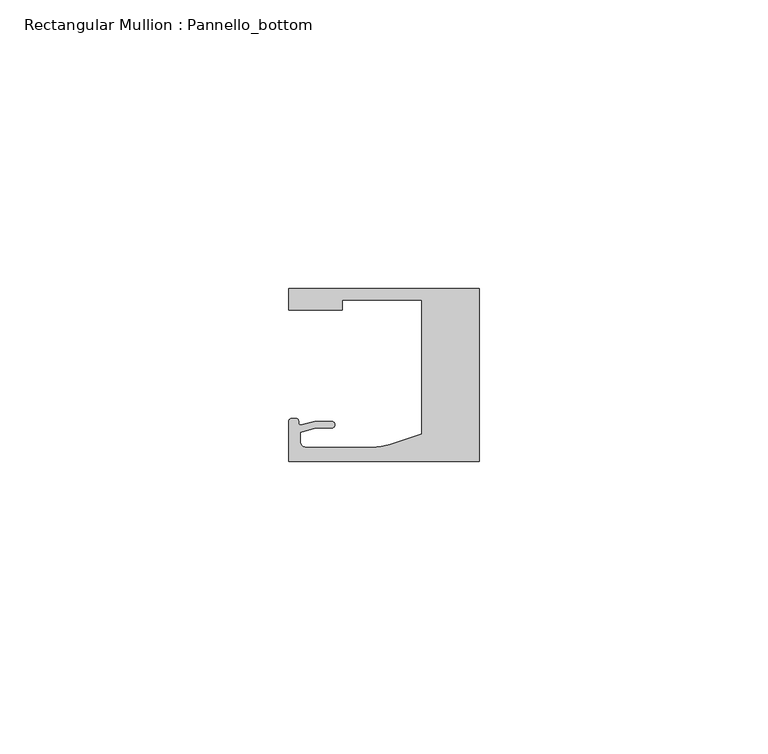
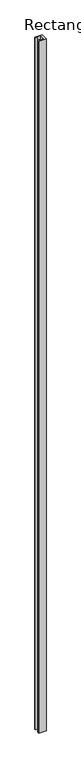
"""IFC4 building model written with IfcOpenShell, lengths in millimetres: member geometry, Rectangular Mullion : Pannello_bottom."""

from ifc_helpers import new_model, si_unit, frame, origin, place, context, project, spatial, polyline, circle_curve, source, transform, mapped, element, save
from ifc_brep_helpers import plane_surface, cylinder_surface, revolved_surface, extruded_surface, spline_curve, advanced_brep


def rectangular_mullion_pannello_bottom_fcb81b7f(model_context):
    return source(origin(), model_context, "Body", "AdvancedBrep", [
        advanced_brep(
        [(-33.0, 15.0, 0.0), (-33.0, 11.3000004, 0.0), (-23.700041, 11.3000004, 0.0), (-23.700041, 13.0000004, 0.0), (-9.9999723, 13.0000004, 0.0), (-9.9999723, -10.2367227, 0.0), (-15.4591336, -12.0105099, 0.0), (-18.5493024, -12.4999438, 0.0), (-30.0000002, -12.4999419, 0.0), (-31.0, -11.4999419, 0.0), (-31.0, -9.9121746, 0.0), (-28.3419477, -9.1999523, 0.0), (-25.59998, -9.1999523, 0.0), (-25.59998, -7.9999523, 0.0), (-28.4999305, -7.9999523, 0.0), (-30.9223017, -8.6490241, 0.0), (-33.0000135, -8.0000472, 0.0), (-33.0000135, -15.0, 0.0), (0.0, -15.0, 0.0), (0.0, 15.0, 0.0), (-33.0, 15.0, -3313.9999729), (0.0, 15.0, -3313.9999729), (0.0, -15.0, -3313.9999729), (-33.0000135, -15.0, -3313.9999729), (-33.0000135, -8.0000472, -3313.9999729), (-30.9223017, -8.6490241, -3313.9999729), (-28.4999305, -7.9999523, -3313.9999729), (-25.59998, -7.9999523, -3313.9999729), (-25.59998, -9.1999523, -3313.9999729), (-28.3419477, -9.1999523, -3313.9999729), (-31.0, -9.9121746, -3313.9999729), (-31.0, -11.4999419, -3313.9999729), (-30.0000002, -12.4999419, -3313.9999729), (-18.5493024, -12.4999438, -3313.9999729), (-15.4591336, -12.0105099, -3313.9999729), (-9.9999723, -10.2367227, -3313.9999729), (-9.9999723, 13.0000004, -3313.9999729), (-23.700041, 13.0000004, -3313.9999729), (-23.700041, 11.3000004, -3313.9999729), (-33.0, 11.3000004, -3313.9999729)],
        [
            (0, 1),
            (1, 2),
            (2, 3),
            (3, 4),
            (4, 5),
            (5, 6),
            (6, 7, circle_curve(frame((-18.5493007, -2.4999438, 0.0), z_axis=(0.0, 0.0, -1.0), x_axis=(0.0, -1.0, 0.0)), 10.0)),
            (7, 8),
            (8, 9, circle_curve(frame((-30.0, -11.4999419, 0.0), z_axis=(0.0, 0.0, -1.0), x_axis=(0.0, -1.0, 0.0)), 1.0)),
            (9, 10),
            (10, 11),
            (11, 12),
            (12, 13, circle_curve(frame((-25.59998, -8.5999523, 0.0), z_axis=(0.0, 0.0, 1.0), x_axis=(0.0, -1.0, 0.0)), 0.6)),
            (13, 14),
            (14, 15),
            (15, 16, spline_curve(3, [(-30.9223017, -8.6490241, 0.0), (-31.312054066, -8.717747958, 0.0), (-31.298563602, -8.366228555, 0.0), (-31.305645054, -7.690065204, 0.0), (-31.357433266, -7.563996614, 0.0), (-32.262327879, -7.456527435, 0.0), (-33.0000135, -7.457047519, 0.0), (-33.0000135, -8.0000472, 0.0)], [4, 2, 2, 4], [0.0, 0.001840817752199412, 0.004996616814974408, 0.007702013405570312])),
            (16, 17),
            (17, 18),
            (18, 19),
            (19, 0),
            (20, 21),
            (21, 22),
            (22, 23),
            (23, 24),
            (24, 25, spline_curve(3, [(-33.0000135, -8.0000472, -3313.9999729), (-33.0000135, -7.457047519, -3313.9999729), (-32.262327879, -7.456527435, -3313.9999729), (-31.357433266, -7.563996614, -3313.9999729), (-31.305645054, -7.690065204, -3313.9999729), (-31.298563602, -8.366228555, -3313.9999729), (-31.312054066, -8.717747958, -3313.9999729), (-30.9223017, -8.6490241, -3313.9999729)], [4, 2, 2, 4], [0.0, 0.0027053965905959043, 0.0058611956533709, 0.007702013405570312])),
            (25, 26),
            (26, 27),
            (27, 28, circle_curve(frame((-25.59998, -8.5999523, -3313.9999729), z_axis=(0.0, 0.0, -1.0), x_axis=(0.0, -1.0, 0.0)), 0.6)),
            (28, 29),
            (29, 30),
            (30, 31),
            (31, 32, circle_curve(frame((-30.0, -11.4999419, -3313.9999729), z_axis=(0.0, 0.0, 1.0), x_axis=(0.0, -1.0, 0.0)), 1.0)),
            (32, 33),
            (33, 34, circle_curve(frame((-18.5493007, -2.4999438, -3313.9999729), z_axis=(0.0, 0.0, 1.0), x_axis=(0.0, -1.0, 0.0)), 10.0)),
            (34, 35),
            (35, 36),
            (36, 37),
            (37, 38),
            (38, 39),
            (39, 20),
            (0, 20),
            (39, 1),
            (38, 2),
            (37, 3),
            (36, 4),
            (35, 5),
            (34, 6),
            (33, 7),
            (32, 8),
            (31, 9),
            (30, 10),
            (29, 11),
            (28, 12),
            (27, 13),
            (26, 14),
            (25, 15),
            (24, 16),
            (23, 17),
            (22, 18),
            (21, 19),
        ],
        [
            plane_surface(frame((0.0, -36.2491502, 0.0), z_axis=(0.0, 0.0, 1.0), x_axis=(-1.0, 0.0, 0.0))),
            plane_surface(frame((0.0, -36.2491502, -3313.9999729), z_axis=(0.0, 0.0, -1.0), x_axis=(-1.0, 0.0, 0.0))),
            plane_surface(frame((-33.0, 15.0, 0.0), z_axis=(-1.0, 0.0, 0.0), x_axis=(0.0, 0.0, -1.0))),
            plane_surface(frame((-33.0, 11.3000004, 0.0), z_axis=(0.0, -1.0, 0.0), x_axis=(0.0, 0.0, -1.0))),
            plane_surface(frame((-23.700041, 11.3000004, 0.0), z_axis=(1.0, 0.0, 0.0), x_axis=(0.0, 0.0, -1.0))),
            plane_surface(frame((-23.700041, 13.0000004, 0.0), z_axis=(0.0, -1.0, 0.0), x_axis=(0.0, 0.0, -1.0))),
            plane_surface(frame((-9.9999723, 13.0000004, 0.0), z_axis=(-1.0, 0.0, 0.0), x_axis=(0.0, 0.0, -1.0))),
            plane_surface(frame((-9.9999723, -10.2367227, 0.0), z_axis=(-0.30901670911956314, 0.9510566089801992, 0.0), x_axis=(0.0, 0.0, -1.0))),
            revolved_surface(polyline([(-18.5493007, -12.4999438, -3313.9999729), (-18.5493007, -12.4999438, 0.0)]), (-18.5493007, -2.4999438, 0.0), (0.0, 0.0, -1.0)),
            plane_surface(frame((-18.5493024, -12.4999438, 0.0), z_axis=(1.6923026533778639e-07, 0.9999999999999858, 0.0), x_axis=(0.0, 0.0, -1.0))),
            revolved_surface(polyline([(-30.0, -12.4999419, -3313.9999729), (-30.0, -12.4999419, 0.0)]), (-30.0, -11.4999419, 0.0), (0.0, 0.0, -1.0)),
            plane_surface(frame((-31.0, -11.4999419, 0.0), z_axis=(1.0, 0.0, 0.0), x_axis=(0.0, 0.0, -1.0))),
            plane_surface(frame((-31.0, -9.9121746, 0.0), z_axis=(0.25881883204288636, -0.9659258833782002, 0.0), x_axis=(0.0, 0.0, -1.0))),
            plane_surface(frame((-28.3419477, -9.1999523, 0.0), z_axis=(0.0, -1.0, 0.0), x_axis=(0.0, 0.0, -1.0))),
            cylinder_surface(frame((-25.59998, -8.5999523, 0.0), z_axis=(0.0, 0.0, 1.0), x_axis=(0.0, -1.0, 0.0)), 0.6),
            plane_surface(frame((-25.59998, -7.9999523, 0.0), z_axis=(0.0, 1.0, 0.0), x_axis=(0.0, 0.0, -1.0))),
            plane_surface(frame((-28.4999305, -7.9999523, 0.0), z_axis=(-0.25881883200192934, 0.9659258833891746, 0.0), x_axis=(0.0, 0.0, -1.0))),
            extruded_surface(spline_curve(3, [(-30.9223017, -8.6490241, -3313.9999729), (-31.312054066, -8.717747958, -3313.9999729), (-31.298563602, -8.366228555, -3313.9999729), (-31.305645054, -7.690065204, -3313.9999729), (-31.357433266, -7.563996614, -3313.9999729), (-32.262327879, -7.456527435, -3313.9999729), (-33.0000135, -7.457047519, -3313.9999729), (-33.0000135, -8.0000472, -3313.9999729)], [4, 2, 2, 4], [0.0, 0.001840817752199412, 0.004996616814974408, 0.007702013405570312]), (0.0, 0.0, 3313.9999729), 3313.9999729),
            plane_surface(frame((-33.0000135, -8.0000472, 0.0), z_axis=(-1.0, 0.0, 0.0), x_axis=(0.0, 0.0, -1.0))),
            plane_surface(frame((-33.0000135, -15.0, 0.0), z_axis=(0.0, -1.0, 0.0), x_axis=(0.0, 0.0, -1.0))),
            plane_surface(frame((0.0, -15.0, 0.0), z_axis=(1.0, 0.0, 0.0), x_axis=(0.0, 0.0, -1.0))),
            plane_surface(frame((0.0, 15.0, 0.0), z_axis=(0.0, 1.0, 0.0), x_axis=(0.0, 0.0, -1.0))),
        ],
        [
            (0, [[1, 2, 3, 4, 5, 6, 7, 8, 9, 10, 11, 12, 13, 14, 15, 16, 17, 18, 19, 20]]),
            (1, [[21, 22, 23, 24, 25, 26, 27, 28, 29, 30, 31, 32, 33, 34, 35, 36, 37, 38, 39, 40]]),
            (2, [[-1, 41, -40, 42]]),
            (3, [[-2, -42, -39, 43]]),
            (4, [[-3, -43, -38, 44]]),
            (5, [[-4, -44, -37, 45]]),
            (6, [[-5, -45, -36, 46]]),
            (7, [[-6, -46, -35, 47]]),
            (8, [[-7, -47, -34, 48]]),
            (9, [[-8, -48, -33, 49]]),
            (10, [[-9, -49, -32, 50]]),
            (11, [[-10, -50, -31, 51]]),
            (12, [[-11, -51, -30, 52]]),
            (13, [[-12, -52, -29, 53]]),
            (14, [[-13, -53, -28, 54]]),
            (15, [[-14, -54, -27, 55]]),
            (16, [[-15, -55, -26, 56]]),
            (17, [[-16, -56, -25, 57]]),
            (18, [[-17, -57, -24, 58]]),
            (19, [[-18, -58, -23, 59]]),
            (20, [[-19, -59, -22, 60]]),
            (21, [[-20, -60, -21, -41]]),
        ],
    ),
    ])


if __name__ == "__main__":
    model = new_model("IFC4")
    model_context = context("Model", 3, world=origin())
    ifc_project = project(units=[si_unit("LENGTHUNIT", "METRE", prefix="MILLI")], contexts=[model_context])
    site = spatial("IfcSite", under=ifc_project)
    building = spatial("IfcBuilding", under=site)
    placement = place(None, origin())
    rectangular_mullion_pannello_bottom_shape = rectangular_mullion_pannello_bottom_fcb81b7f(model_context)
    element("IfcMember", 1, ObjectType="Rectangular Mullion : Pannello_bottom", at=placement, inside=building, context=model_context, shape_type="MappedRepresentation", body=[
        mapped(rectangular_mullion_pannello_bottom_shape, transform((0.0, 0.0, 0.0), x_axis=(1.0, 0.0, 0.0), y_axis=(0.0, 1.0, 0.0), z_axis=(0.0, 0.0, 1.0))),
    ])
    save(model, "model.ifc")

# Revit data of these elements
# Type "Rectangular Mullion : Pannello_bottom"
#   built-in parameter 1007322 = 0.0984252 (stored number, unit not read)
#   built-in parameter 1007321 = 0.0328083 (stored number, unit not read)
#   built-in parameter 1007320 = 0 (stored number, unit not read)
